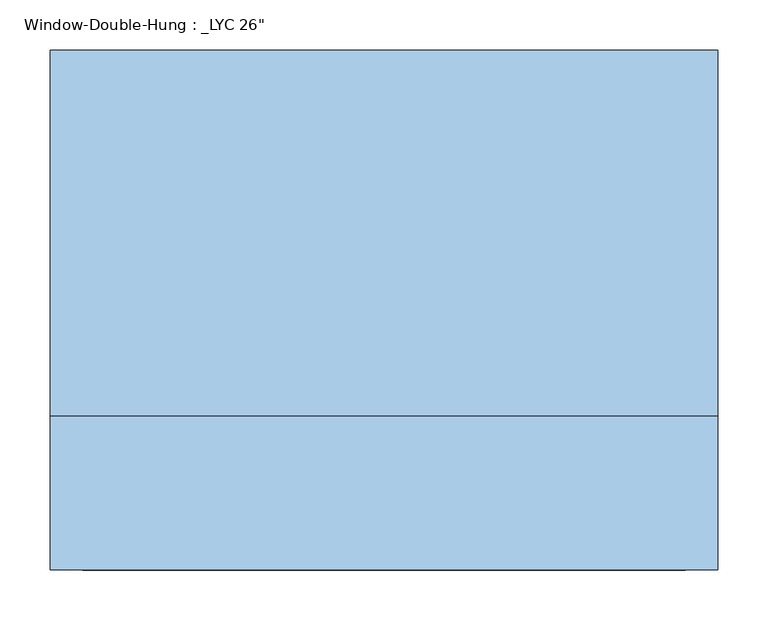
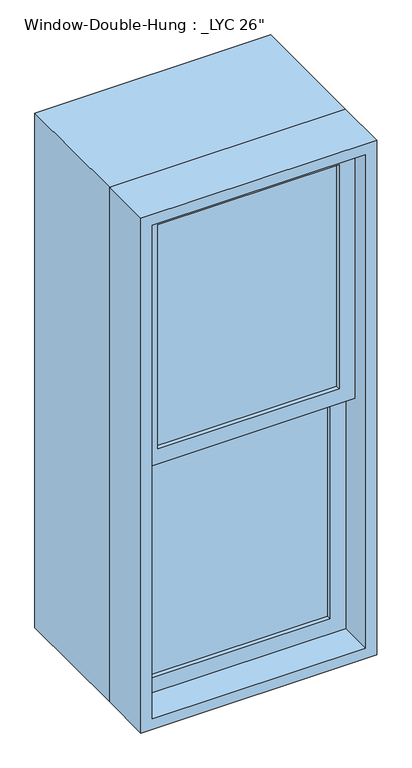
"""IFC4 building model written with IfcOpenShell, lengths in millimetres: window geometry."""

from ifc_helpers import new_model, si_unit, frame, origin, place, context, project, spatial, polyline, outline, extrude, source, transform, mapped, element, save


def window_16a2ee0f(model_context):
    return source(origin(), model_context, "Body", "SweptSolid", [
        extrude(outline(polyline([(254.0, -158.75), (-254.0, -158.75), (-254.0, -152.4), (254.0, -152.4), (254.0, -158.75)])), frame((0.0, 0.0, 990.6), z_axis=(0.0, 0.0, 1.0), x_axis=(1.0, 0.0, 0.0)), (0.0, 0.0, 1.0), 663.575),
        extrude(outline(polyline([(-254.0, -146.05), (-254.0, -139.7), (254.0, -139.7), (254.0, -146.05), (-254.0, -146.05)])), frame((0.0, 0.0, 990.6), z_axis=(0.0, 0.0, 1.0), x_axis=(1.0, 0.0, 0.0)), (0.0, 0.0, 1.0), 663.575),
        extrude(outline(polyline([(254.0, -203.2), (-254.0, -203.2), (-254.0, -196.85), (254.0, -196.85), (254.0, -203.2)])), frame((0.0, 0.0, 1698.625), z_axis=(0.0, 0.0, 1.0), x_axis=(1.0, 0.0, 0.0)), (0.0, 0.0, 1.0), 663.575),
        extrude(outline(polyline([(-254.0, -190.5), (-254.0, -184.15), (254.0, -184.15), (254.0, -190.5), (-254.0, -190.5)])), frame((0.0, 0.0, 1698.625), z_axis=(0.0, 0.0, 1.0), x_axis=(1.0, 0.0, 0.0)), (0.0, 0.0, 1.0), 663.575),
        extrude(outline(polyline([(1698.625, 298.45), (1698.625, -298.45), (946.15, -298.45), (946.15, 298.45), (1698.625, 298.45)]), holes=[polyline([(1654.175, -254.0), (1654.175, 254.0), (990.6, 254.0), (990.6, -254.0), (1654.175, -254.0)])]), frame((0.0, -171.45, 0.0), z_axis=(0.0, 1.0, 0.0), x_axis=(0.0, 0.0, 1.0)), (0.0, 0.0, 1.0), 44.45),
        extrude(outline(polyline([(2406.65, 298.45), (2406.65, -298.45), (1654.175, -298.45), (1654.175, 298.45), (2406.65, 298.45)]), holes=[polyline([(2362.2, -254.0), (2362.2, 254.0), (1698.625, 254.0), (1698.625, -254.0), (2362.2, -254.0)])]), frame((0.0, -215.9, 0.0), z_axis=(0.0, 1.0, 0.0), x_axis=(0.0, 0.0, 1.0)), (0.0, 0.0, 1.0), 44.45),
        extrude(outline(polyline([(2438.4, 330.2), (2438.4, -330.2), (914.4, -330.2), (914.4, 330.2), (2438.4, 330.2)]), holes=[polyline([(2406.65, -298.45), (2406.65, 298.45), (946.15, 298.45), (946.15, -298.45), (2406.65, -298.45)])]), frame((0.0, -266.7, 0.0), z_axis=(0.0, 1.0, 0.0), x_axis=(0.0, 0.0, 1.0)), (0.0, 0.0, 1.0), 152.4),
        extrude(outline(polyline([(2438.4, 330.2), (2438.4, -330.2), (914.4, -330.2), (914.4, 330.2), (2438.4, 330.2)]), holes=[polyline([(2419.35, 311.15), (933.45, 311.15), (933.45, -311.15), (2419.35, -311.15), (2419.35, 311.15)])]), frame((0.0, -114.3, 0.0), z_axis=(0.0, 1.0, 0.0), x_axis=(0.0, 0.0, 1.0)), (0.0, 0.0, 1.0), 361.95),
    ])


if __name__ == "__main__":
    model = new_model("IFC4")
    model_context = context("Model", 3, world=origin())
    ifc_project = project(units=[si_unit("LENGTHUNIT", "METRE", prefix="MILLI")], contexts=[model_context])
    site = spatial("IfcSite", under=ifc_project)
    building = spatial("IfcBuilding", under=site)
    placement = place(None, origin())
    window_shape = window_16a2ee0f(model_context)
    element("IfcWindow", 1, ObjectType="Window-Double-Hung : _LYC 26\"", at=placement, inside=building, context=model_context, shape_type="MappedRepresentation", body=[
        mapped(window_shape, transform((0.0, 0.0, 0.0), x_axis=(1.0, 0.0, 0.0), y_axis=(0.0, 1.0, 0.0), z_axis=(0.0, 0.0, 1.0))),
    ])
    save(model, "model.ifc")

# Revit data of these elements
# Type "Window-Double-Hung : _LYC 26\""
#   Type Mark = "21"
#   Fire Rating = "0.5h"
#   Assembly Code = "B2020100"
#   Wall Thickness [instance default] = 0' - 6"
#   Visual Light Transmittance = 0.9
#   Thermal Resistance (R) = 1.8146 (h·ft²·°F)/BTU
#   Solar Heat Gain Coefficient = 0.78
#   Rough Width = 2' - 2 1/2"
#   Rough Height = 5' - 0 1/2"
#   Muntin Width = 1' - 8"
#   Muntin Height = 2' - 2 1/8"
#   Interior Wall Closure [instance default] = 0' - 1 1/2"
#   Heat Transfer Coefficient (U) = 0.6496 BTU/(h·ft²·°F)
#   Frame Extension [instance default] = 0' - 2"
#   Exterior Wall Closure [instance default] = 0' - 0 1/2"
#   Extension Jamb [instance default] = 0' - 0 3/4"
#   Height = 5' - 0"
#   Width = 2' - 2"
#   Window Inset [instance default] = 0' - 0 3/4"
#   Top Muntin Visibility = yes
#   Interior Trim Visibility [instance default] = yes
#   Indicator Visibility [instance default] = yes
#   Exterior Trim Visibility [instance default] = yes
#   Extension Jamb Visibility [instance default] = yes
#   Define Thermal Properties by = 1
#   Bottom Muntin Visibility = yes
#   Muntin Pattern = Muntin Pattern_2x2 : Muntin Pattern_2x2
#   Interior Trim Material = Wood - Stained
#   Interior Trim = Trim-Window-Interior-Flat : Picture Frame
#   Interior Frame Material = Wood - Stained
#   Glass Panel Material = Glass
#   Exterior Trim Material = Clad - White
#   Exterior Trim = Trim-Window-Exterior-Flat : with Sill
#   Exterior Frame Material = Clad - White
#   Construction Type Id = ""
#   Wall Closure = (empty or 0)
#   Analytic Construction = (empty or 0)
# Element 1 (IfcWindow, "Window-Double-Hung : _LYC 26\"")
#   Wall Thickness = 1' - 7 1/2"
#   Extension Jamb = 1' - 2 1/4"
#   Materials on its faces: "Wood - Stained", "Glass", "Clad - White"
# Materials
#   "Wood - Stained": class "Wood", colour RGB 224 178 126, transparency 0, Cost = 0
#   "Glass": class "Unassigned", colour RGB 0 128 192, transparency 0.75
#   "Clad - White": class "Wood", colour RGB 242 242 238, transparency 0, Cost = 0
